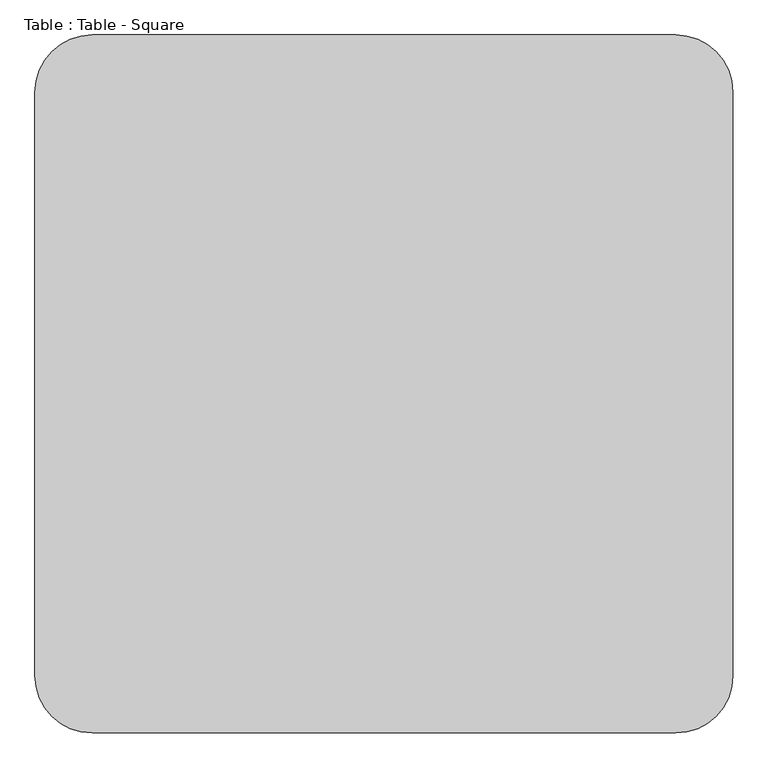
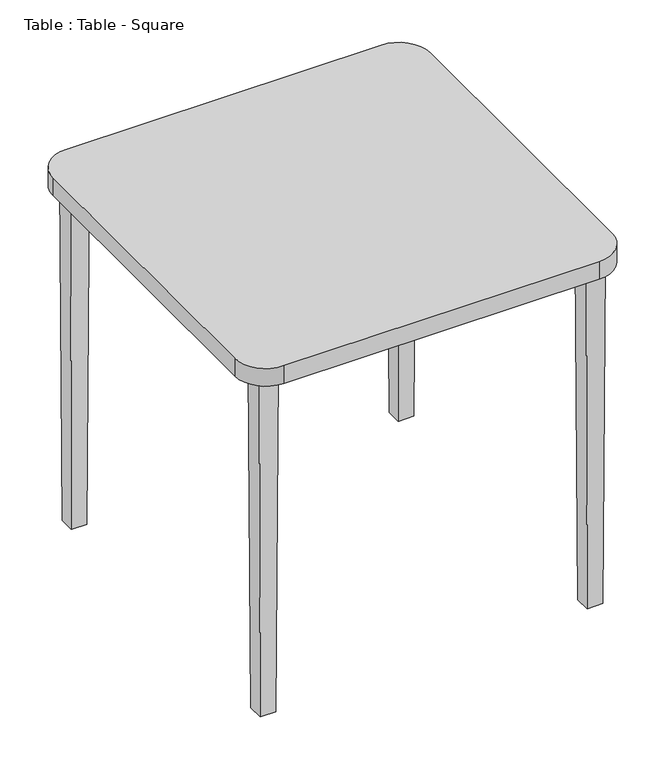
"""IFC4 building model written with IfcOpenShell, lengths in millimetres: proxy geometry, Table : Table - Square."""

import ifcopenshell
import ifcopenshell.guid

model = None  # the IFC model being written
_history = None  # IfcOwnerHistory: only IFC2X3 demands one
_inside = {}  # id of a spatial element -> (the spatial element, [elements in it])
_under = {}  # id of a project, library or spatial element -> (it, [spatial elements below it])
_declared = {}  # id of a project -> (the project, [libraries it declares])
_typed = {}  # id of a type object -> (the type object, [elements of that type])
_made_of = {}  # id of a material, layer set ... -> (it, [elements and type objects made of it])


def new_model(schema):
    """Start an empty IFC model of exactly this schema.

    Asked for "IFC4X3", IfcOpenShell would pick the latest addendum, in which some entities
    have other attributes; the version numbers below select the first issue.
    IFC2X3 requires an IfcOwnerHistory on every rooted entity: one is made here for all.
    """
    global model, _history
    if schema == "IFC4X3":
        model = ifcopenshell.file(schema_version=(4, 3, 0, 0))
    else:
        model = ifcopenshell.file(schema=schema)
    _inside.clear()
    _under.clear()
    _declared.clear()
    _typed.clear()
    _made_of.clear()
    _history = None
    if model.schema == "IFC2X3":
        org = make("IfcOrganization", Name="unknown")
        user = make(
            "IfcPersonAndOrganization",
            ThePerson=make("IfcPerson", FamilyName="unknown"),
            TheOrganization=org,
        )
        app = make(
            "IfcApplication",
            ApplicationDeveloper=org,
            Version="unknown",
            ApplicationFullName="unknown",
            ApplicationIdentifier="unknown",
        )
        _history = make(
            "IfcOwnerHistory",
            OwningUser=user,
            OwningApplication=app,
            ChangeAction="ADDED",
            CreationDate=0,
        )
    return model


def make(cls, **values):
    """One entity of the class cls with the attributes given. An attribute that is None is left unset."""
    return model.create_entity(
        cls, **{name: value for name, value in values.items() if value is not None}
    )


def rooted(cls, **values):
    """An entity with a GlobalId (a new one), such as an element, a storey or a relation."""
    return make(cls, GlobalId=ifcopenshell.guid.new(), OwnerHistory=_history, **values)


def si_unit(unit_type, name, prefix=None):
    """IfcSIUnit, for example si_unit("LENGTHUNIT", "METRE", prefix="MILLI")."""
    return make("IfcSIUnit", UnitType=unit_type, Prefix=prefix, Name=name)


def assignment(units):
    """IfcUnitAssignment: the units of a project."""
    return None if units is None else make("IfcUnitAssignment", Units=units)


def point(xyz):
    """IfcCartesianPoint."""
    return None if xyz is None else make("IfcCartesianPoint", Coordinates=xyz)


def direction(xyz):
    """IfcDirection."""
    return None if xyz is None else make("IfcDirection", DirectionRatios=xyz)


def frame(location, z_axis=None, x_axis=None):
    """IfcAxis2Placement3D, a coordinate frame: its origin and axes. An axis left out is left unset."""
    return make(
        "IfcAxis2Placement3D",
        Location=point(location),
        Axis=direction(z_axis),
        RefDirection=direction(x_axis),
    )


def frame_2d(location, x_axis=None):
    """IfcAxis2Placement2D, a coordinate frame in the plane: its origin and x axis."""
    return make(
        "IfcAxis2Placement2D", Location=point(location), RefDirection=direction(x_axis)
    )


def origin():
    """The frame at (0, 0, 0) with its axes left unset."""
    return frame((0.0, 0.0, 0.0))


def place(relative_to, where):
    """IfcLocalPlacement: puts the frame where relative to a parent placement (None: the world)."""
    return make(
        "IfcLocalPlacement", PlacementRelTo=relative_to, RelativePlacement=where
    )


def context(
    kind, dimensions, precision=None, world=None, true_north=None, identifier=None
):
    """IfcGeometricRepresentationContext, for example the 3D "Model" context."""
    return make(
        "IfcGeometricRepresentationContext",
        ContextIdentifier=identifier,
        ContextType=kind,
        CoordinateSpaceDimension=dimensions,
        Precision=precision,
        WorldCoordinateSystem=world,
        TrueNorth=true_north,
    )


def project(units=None, contexts=None):
    """IfcProject with its units and contexts."""
    return rooted(
        "IfcProject",
        Name="project",
        RepresentationContexts=contexts,
        UnitsInContext=assignment(units),
    )


def spatial(cls, under=None, at=None, **own):
    """A site, building, storey or space (cls), placed at a placement, below another one or the project."""
    s = rooted(cls, ObjectPlacement=at, **own)
    if under is not None:
        _under.setdefault(under.id(), (under, []))[1].append(s)
    return s


def polyline(points):
    """IfcPolyline through the points."""
    return make("IfcPolyline", Points=[point(p) for p in points])


def circle_curve(where, radius):
    """IfcCircle in the frame where."""
    return make("IfcCircle", Position=where, Radius=radius)


def trimmed(basis, trim1, trim2, sense, master):
    """IfcTrimmedCurve: the piece of a basis curve between two trims."""
    return make(
        "IfcTrimmedCurve",
        BasisCurve=basis,
        Trim1=trim1,
        Trim2=trim2,
        SenseAgreement=sense,
        MasterRepresentation=master,
    )


def segment(curve, same_sense, transition):
    """IfcCompositeCurveSegment."""
    return make(
        "IfcCompositeCurveSegment",
        Transition=transition,
        SameSense=same_sense,
        ParentCurve=curve,
    )


def composite_curve(segments, self_intersect=None):
    """IfcCompositeCurve: segments joined end to end."""
    return make("IfcCompositeCurve", Segments=segments, SelfIntersect=self_intersect)


def outline(outer, holes=None, kind="AREA"):
    """IfcArbitraryClosedProfileDef: a profile drawn as a closed curve; with holes, ...WithVoids."""
    if holes is None:
        return make("IfcArbitraryClosedProfileDef", ProfileType=kind, OuterCurve=outer)
    return make(
        "IfcArbitraryProfileDefWithVoids",
        ProfileType=kind,
        OuterCurve=outer,
        InnerCurves=holes,
    )


def extrude(swept, where, along, depth):
    """IfcExtrudedAreaSolid: the profile swept, set in the frame where, extruded along a direction by depth."""
    return make(
        "IfcExtrudedAreaSolid",
        SweptArea=swept,
        Position=where,
        ExtrudedDirection=direction(along),
        Depth=depth,
    )


def faces_of(points, faces, orient=None, outer=None):
    """IfcFace entities. A face is a list of loops; a loop is a list of indices into points, from 0.

    orient and outer hold one flag for each loop. By default every Orientation is true, the
    first loop of a face is its IfcFaceOuterBound and the others are IfcFaceBound.
    """
    made = []
    for i, loops in enumerate(faces):
        bounds = []
        for j, loop in enumerate(loops):
            is_outer = j == 0 if outer is None else outer[i][j]
            bounds.append(
                make(
                    "IfcFaceOuterBound" if is_outer else "IfcFaceBound",
                    Bound=make("IfcPolyLoop", Polygon=[points[k] for k in loop]),
                    Orientation=True if orient is None else orient[i][j],
                )
            )
        made.append(make("IfcFace", Bounds=bounds))
    return made


def faceted_brep(points, faces, orient=None, outer=None, voids=None):
    """IfcFacetedBrep: a solid bounded by flat faces; with voids (closed shells), ...WithVoids."""
    shared = [point(p) for p in points]
    hull = make("IfcClosedShell", CfsFaces=faces_of(shared, faces, orient, outer))
    if voids is None:
        return make("IfcFacetedBrep", Outer=hull)
    return make(
        "IfcFacetedBrepWithVoids",
        Outer=hull,
        Voids=[
            make(cls, CfsFaces=faces_of(shared, fs, o, b)) for cls, fs, o, b in voids
        ],
    )


def shape(context_of_items, identifier, shape_type, items):
    """IfcShapeRepresentation: the items that make up one representation, for example the "Body"."""
    return make(
        "IfcShapeRepresentation",
        ContextOfItems=context_of_items,
        RepresentationIdentifier=identifier,
        RepresentationType=shape_type,
        Items=items,
    )


def source(mapping_origin, context_of_items, identifier, shape_type, items):
    """IfcRepresentationMap: a shape defined once, which mapped items show again and again."""
    return make(
        "IfcRepresentationMap",
        MappingOrigin=mapping_origin,
        MappedRepresentation=shape(context_of_items, identifier, shape_type, items),
    )


def transform(
    local_origin,
    x_axis=None,
    y_axis=None,
    z_axis=None,
    scale=None,
    scale2=None,
    scale3=None,
    uniform=True,
):
    """IfcCartesianTransformationOperator3D, or its non-uniform kind. x_axis, y_axis, z_axis: its Axis1, 2, 3."""
    if uniform:
        return make(
            "IfcCartesianTransformationOperator3D",
            Axis1=direction(x_axis),
            Axis2=direction(y_axis),
            LocalOrigin=point(local_origin),
            Scale=scale,
            Axis3=direction(z_axis),
        )
    return make(
        "IfcCartesianTransformationOperator3DnonUniform",
        Axis1=direction(x_axis),
        Axis2=direction(y_axis),
        LocalOrigin=point(local_origin),
        Scale=scale,
        Axis3=direction(z_axis),
        Scale2=scale2,
        Scale3=scale3,
    )


def mapped(mapping_source, mapping_target):
    """IfcMappedItem: shows the shape of a source again, moved by a transform."""
    return make(
        "IfcMappedItem", MappingSource=mapping_source, MappingTarget=mapping_target
    )


def made_of(thing, what):
    """Note that an element or type object is made of a material, layer set ...; save() writes the relation."""
    if what is not None:
        _made_of.setdefault(what.id(), (what, []))[1].append(thing)
    return thing


def element(
    cls,
    number,
    at=None,
    inside=None,
    cuts=None,
    type_object=None,
    material=None,
    context=None,
    identifier="Body",
    shape_type=None,
    held_by="IfcProductDefinitionShape",
    body=None,
    shapes=None,
    **own,
):
    """One element of the class cls, such as IfcWall. Its Tag is "e" and its number.

    at: its placement. inside: the storey or other place that contains it. cuts: it is an
    opening in that element (IfcRelVoidsElement). A single representation is given by context,
    identifier, shape_type and body (its items); several are given by shapes. held_by: the class
    of the entity that holds the representations. save() writes the other relations.
    """
    e = rooted(cls, Tag="e%d" % number, ObjectPlacement=at, **own)
    if body is not None:
        shapes = [shape(context, identifier, shape_type, body)]
    if shapes is not None:
        e.Representation = make(held_by, Representations=shapes)
    if inside is not None:
        _inside.setdefault(inside.id(), (inside, []))[1].append(e)
    if cuts is not None:
        rooted(
            "IfcRelVoidsElement", RelatingBuildingElement=cuts, RelatedOpeningElement=e
        )
    if type_object is not None:
        _typed.setdefault(type_object.id(), (type_object, []))[1].append(e)
    return made_of(e, material)


def aggregate(whole, parts):
    """IfcRelAggregates: a whole, such as a stair, and the parts it consists of."""
    return rooted("IfcRelAggregates", RelatingObject=whole, RelatedObjects=parts)


def save(model, path):
    """Write the relations noted so far, then the file.

    IfcRelAggregates (storeys below a building ...), IfcRelContainedInSpatialStructure (elements
    in a storey), IfcRelDefinesByType, IfcRelAssociatesMaterial and IfcRelDeclares: one each for
    every whole, place, type object, material and project.
    """
    for whole, parts in _under.values():
        aggregate(whole, parts)
    for where, things in _inside.values():
        rooted(
            "IfcRelContainedInSpatialStructure",
            RelatedElements=things,
            RelatingStructure=where,
        )
    for kind, things in _typed.values():
        rooted("IfcRelDefinesByType", RelatedObjects=things, RelatingType=kind)
    for what, things in _made_of.values():
        rooted("IfcRelAssociatesMaterial", RelatedObjects=things, RelatingMaterial=what)
    for by, libraries in _declared.values():
        rooted("IfcRelDeclares", RelatingContext=by, RelatedDefinitions=libraries)
    model.write(path)


def table_table_square_88d88849(model_context):
    return source(origin(), model_context, "Body", "SolidModel", [
        faceted_brep([(-622.3, -622.3, 1447.8), (-698.5, -622.3, 1447.8), (-698.5, -698.5, 1447.8), (-622.3, -698.5, 1447.8), (-628.65, -628.65, 0.0), (-628.65, -692.15, 0.0), (-692.15, -692.15, 0.0), (-692.15, -628.65, 0.0)], [[[0, 1, 2, 3]], [[4, 5, 6, 7]], [[4, 7, 1, 0]], [[7, 6, 2, 1]], [[6, 5, 3, 2]], [[5, 4, 0, 3]]]),
        faceted_brep([(698.5, -622.3, 1447.8), (622.3, -622.3, 1447.8), (622.3, -698.5, 1447.8), (698.5, -698.5, 1447.8), (692.15, -628.65, 0.0), (692.15, -692.15, 0.0), (628.65, -692.15, 0.0), (628.65, -628.65, 0.0)], [[[0, 1, 2, 3]], [[4, 5, 6, 7]], [[4, 7, 1, 0]], [[7, 6, 2, 1]], [[6, 5, 3, 2]], [[5, 4, 0, 3]]]),
        faceted_brep([(698.5, 698.5, 1447.8), (622.3, 698.5, 1447.8), (622.3, 622.3, 1447.8), (698.5, 622.3, 1447.8), (692.15, 692.15, 0.0), (692.15, 628.65, 0.0), (628.65, 628.65, 0.0), (628.65, 692.15, 0.0)], [[[0, 1, 2, 3]], [[4, 5, 6, 7]], [[4, 7, 1, 0]], [[7, 6, 2, 1]], [[6, 5, 3, 2]], [[5, 4, 0, 3]]]),
        faceted_brep([(-622.3, 698.5, 1447.8), (-698.5, 698.5, 1447.8), (-698.5, 622.3, 1447.8), (-622.3, 622.3, 1447.8), (-628.65, 692.15, 0.0), (-628.65, 628.65, 0.0), (-692.15, 628.65, 0.0), (-692.15, 692.15, 0.0)], [[[0, 1, 2, 3]], [[4, 5, 6, 7]], [[4, 7, 1, 0]], [[7, 6, 2, 1]], [[6, 5, 3, 2]], [[5, 4, 0, 3]]]),
        extrude(outline(composite_curve([segment(trimmed(circle_curve(frame_2d((637.032, 637.032)), 124.968), [point((637.032, 762.0))], [point((762.0, 637.032))], False, "CARTESIAN"), True, "CONTINUOUS"), segment(polyline([(762.0, 637.032), (762.0, -637.032)]), True, "CONTINUOUS"), segment(trimmed(circle_curve(frame_2d((637.032, -637.032)), 124.968), [point((762.0, -637.032))], [point((637.032, -762.0))], False, "CARTESIAN"), True, "CONTINUOUS"), segment(polyline([(637.032, -762.0), (-637.032, -762.0)]), True, "CONTINUOUS"), segment(trimmed(circle_curve(frame_2d((-637.032, -637.032)), 124.968), [point((-637.032, -762.0))], [point((-762.0, -637.032))], False, "CARTESIAN"), True, "CONTINUOUS"), segment(polyline([(-762.0, -637.032), (-762.0, 637.032)]), True, "CONTINUOUS"), segment(trimmed(circle_curve(frame_2d((-637.032, 637.032)), 124.968), [point((-762.0, 637.032))], [point((-637.032, 762.0))], False, "CARTESIAN"), True, "CONTINUOUS"), segment(polyline([(-637.032, 762.0), (637.032, 762.0)]), True, "CONTINUOUS")], self_intersect=False)), frame((0.0, 0.0, 1447.8), z_axis=(0.0, 0.0, 1.0), x_axis=(1.0, 0.0, 0.0)), (0.0, 0.0, 1.0), 76.2),
    ])


if __name__ == "__main__":
    model = new_model("IFC4")
    model_context = context("Model", 3, world=origin())
    ifc_project = project(units=[si_unit("LENGTHUNIT", "METRE", prefix="MILLI")], contexts=[model_context])
    site = spatial("IfcSite", under=ifc_project)
    building = spatial("IfcBuilding", under=site)
    placement = place(None, origin())
    table_table_square_shape = table_table_square_88d88849(model_context)
    element("IfcBuildingElementProxy", 1, Name="Table : Table - Square", ObjectType="Table : Table - Square", at=placement, inside=building, context=model_context, shape_type="MappedRepresentation", body=[
        mapped(table_table_square_shape, transform((0.0, 0.0, 0.0), x_axis=(1.0, 0.0, 0.0), y_axis=(0.0, 1.0, 0.0), z_axis=(0.0, 0.0, 1.0))),
    ])
    save(model, "model.ifc")

# Revit data of these elements
# Type "Table : Table - Square"
#   Thickness [instance default] = 0' - 2"
#   Sides [instance default] = 3' - 0"
#   Leg Inset [instance default] = 0' - 4"
#   Leg Height [instance default] = 5' - 8"
#   Height [instance default] = 5' - 10"
#   Corner Fillet [instance default] = 0' - 4"
#   Default Elevation = 0
# Element 1 (IfcBuildingElementProxy, "Table : Table - Square")
#   Thickness = 0' - 3"
#   Sides = 5' - 0"
#   Leg Height = 4' - 9"
#   Height = 5' - 0"
#   Corner Fillet = 0' - 4.92"
